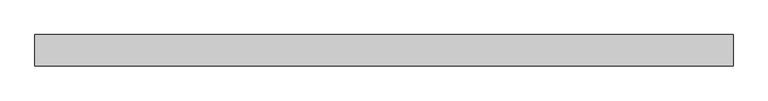
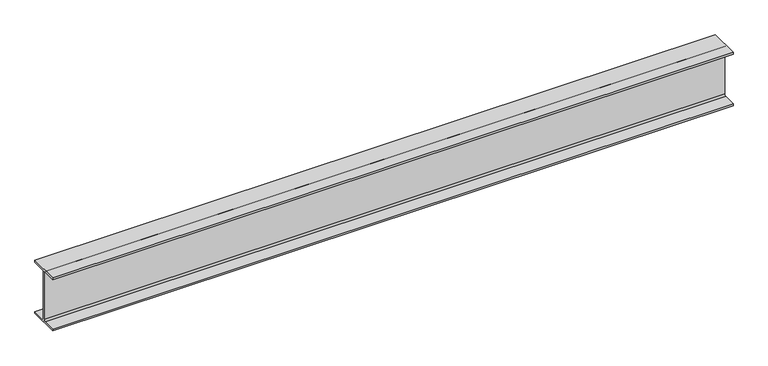
"""IFC4 building model written with IfcOpenShell, lengths in millimetres: beam geometry, Steel Beam_H-KSD3502 : H_SB_ASB_H-200x200x8x12."""

import ifcopenshell
import ifcopenshell.guid

model = None  # the IFC model being written
_history = None  # IfcOwnerHistory: only IFC2X3 demands one
_inside = {}  # id of a spatial element -> (the spatial element, [elements in it])
_under = {}  # id of a project, library or spatial element -> (it, [spatial elements below it])
_declared = {}  # id of a project -> (the project, [libraries it declares])
_typed = {}  # id of a type object -> (the type object, [elements of that type])
_made_of = {}  # id of a material, layer set ... -> (it, [elements and type objects made of it])


def new_model(schema):
    """Start an empty IFC model of exactly this schema.

    Asked for "IFC4X3", IfcOpenShell would pick the latest addendum, in which some entities
    have other attributes; the version numbers below select the first issue.
    IFC2X3 requires an IfcOwnerHistory on every rooted entity: one is made here for all.
    """
    global model, _history
    if schema == "IFC4X3":
        model = ifcopenshell.file(schema_version=(4, 3, 0, 0))
    else:
        model = ifcopenshell.file(schema=schema)
    _inside.clear()
    _under.clear()
    _declared.clear()
    _typed.clear()
    _made_of.clear()
    _history = None
    if model.schema == "IFC2X3":
        org = make("IfcOrganization", Name="unknown")
        user = make(
            "IfcPersonAndOrganization",
            ThePerson=make("IfcPerson", FamilyName="unknown"),
            TheOrganization=org,
        )
        app = make(
            "IfcApplication",
            ApplicationDeveloper=org,
            Version="unknown",
            ApplicationFullName="unknown",
            ApplicationIdentifier="unknown",
        )
        _history = make(
            "IfcOwnerHistory",
            OwningUser=user,
            OwningApplication=app,
            ChangeAction="ADDED",
            CreationDate=0,
        )
    return model


def make(cls, **values):
    """One entity of the class cls with the attributes given. An attribute that is None is left unset."""
    return model.create_entity(
        cls, **{name: value for name, value in values.items() if value is not None}
    )


def rooted(cls, **values):
    """An entity with a GlobalId (a new one), such as an element, a storey or a relation."""
    return make(cls, GlobalId=ifcopenshell.guid.new(), OwnerHistory=_history, **values)


def si_unit(unit_type, name, prefix=None):
    """IfcSIUnit, for example si_unit("LENGTHUNIT", "METRE", prefix="MILLI")."""
    return make("IfcSIUnit", UnitType=unit_type, Prefix=prefix, Name=name)


def assignment(units):
    """IfcUnitAssignment: the units of a project."""
    return None if units is None else make("IfcUnitAssignment", Units=units)


def point(xyz):
    """IfcCartesianPoint."""
    return None if xyz is None else make("IfcCartesianPoint", Coordinates=xyz)


def direction(xyz):
    """IfcDirection."""
    return None if xyz is None else make("IfcDirection", DirectionRatios=xyz)


def frame(location, z_axis=None, x_axis=None):
    """IfcAxis2Placement3D, a coordinate frame: its origin and axes. An axis left out is left unset."""
    return make(
        "IfcAxis2Placement3D",
        Location=point(location),
        Axis=direction(z_axis),
        RefDirection=direction(x_axis),
    )


def frame_2d(location, x_axis=None):
    """IfcAxis2Placement2D, a coordinate frame in the plane: its origin and x axis."""
    return make(
        "IfcAxis2Placement2D", Location=point(location), RefDirection=direction(x_axis)
    )


def origin():
    """The frame at (0, 0, 0) with its axes left unset."""
    return frame((0.0, 0.0, 0.0))


def place(relative_to, where):
    """IfcLocalPlacement: puts the frame where relative to a parent placement (None: the world)."""
    return make(
        "IfcLocalPlacement", PlacementRelTo=relative_to, RelativePlacement=where
    )


def context(
    kind, dimensions, precision=None, world=None, true_north=None, identifier=None
):
    """IfcGeometricRepresentationContext, for example the 3D "Model" context."""
    return make(
        "IfcGeometricRepresentationContext",
        ContextIdentifier=identifier,
        ContextType=kind,
        CoordinateSpaceDimension=dimensions,
        Precision=precision,
        WorldCoordinateSystem=world,
        TrueNorth=true_north,
    )


def project(units=None, contexts=None):
    """IfcProject with its units and contexts."""
    return rooted(
        "IfcProject",
        Name="project",
        RepresentationContexts=contexts,
        UnitsInContext=assignment(units),
    )


def spatial(cls, under=None, at=None, **own):
    """A site, building, storey or space (cls), placed at a placement, below another one or the project."""
    s = rooted(cls, ObjectPlacement=at, **own)
    if under is not None:
        _under.setdefault(under.id(), (under, []))[1].append(s)
    return s


def polyline(points):
    """IfcPolyline through the points."""
    return make("IfcPolyline", Points=[point(p) for p in points])


def circle_curve(where, radius):
    """IfcCircle in the frame where."""
    return make("IfcCircle", Position=where, Radius=radius)


def trimmed(basis, trim1, trim2, sense, master):
    """IfcTrimmedCurve: the piece of a basis curve between two trims."""
    return make(
        "IfcTrimmedCurve",
        BasisCurve=basis,
        Trim1=trim1,
        Trim2=trim2,
        SenseAgreement=sense,
        MasterRepresentation=master,
    )


def segment(curve, same_sense, transition):
    """IfcCompositeCurveSegment."""
    return make(
        "IfcCompositeCurveSegment",
        Transition=transition,
        SameSense=same_sense,
        ParentCurve=curve,
    )


def composite_curve(segments, self_intersect=None):
    """IfcCompositeCurve: segments joined end to end."""
    return make("IfcCompositeCurve", Segments=segments, SelfIntersect=self_intersect)


def outline(outer, holes=None, kind="AREA"):
    """IfcArbitraryClosedProfileDef: a profile drawn as a closed curve; with holes, ...WithVoids."""
    if holes is None:
        return make("IfcArbitraryClosedProfileDef", ProfileType=kind, OuterCurve=outer)
    return make(
        "IfcArbitraryProfileDefWithVoids",
        ProfileType=kind,
        OuterCurve=outer,
        InnerCurves=holes,
    )


def extrude(swept, where, along, depth):
    """IfcExtrudedAreaSolid: the profile swept, set in the frame where, extruded along a direction by depth."""
    return make(
        "IfcExtrudedAreaSolid",
        SweptArea=swept,
        Position=where,
        ExtrudedDirection=direction(along),
        Depth=depth,
    )


def shape(context_of_items, identifier, shape_type, items):
    """IfcShapeRepresentation: the items that make up one representation, for example the "Body"."""
    return make(
        "IfcShapeRepresentation",
        ContextOfItems=context_of_items,
        RepresentationIdentifier=identifier,
        RepresentationType=shape_type,
        Items=items,
    )


def source(mapping_origin, context_of_items, identifier, shape_type, items):
    """IfcRepresentationMap: a shape defined once, which mapped items show again and again."""
    return make(
        "IfcRepresentationMap",
        MappingOrigin=mapping_origin,
        MappedRepresentation=shape(context_of_items, identifier, shape_type, items),
    )


def transform(
    local_origin,
    x_axis=None,
    y_axis=None,
    z_axis=None,
    scale=None,
    scale2=None,
    scale3=None,
    uniform=True,
):
    """IfcCartesianTransformationOperator3D, or its non-uniform kind. x_axis, y_axis, z_axis: its Axis1, 2, 3."""
    if uniform:
        return make(
            "IfcCartesianTransformationOperator3D",
            Axis1=direction(x_axis),
            Axis2=direction(y_axis),
            LocalOrigin=point(local_origin),
            Scale=scale,
            Axis3=direction(z_axis),
        )
    return make(
        "IfcCartesianTransformationOperator3DnonUniform",
        Axis1=direction(x_axis),
        Axis2=direction(y_axis),
        LocalOrigin=point(local_origin),
        Scale=scale,
        Axis3=direction(z_axis),
        Scale2=scale2,
        Scale3=scale3,
    )


def mapped(mapping_source, mapping_target):
    """IfcMappedItem: shows the shape of a source again, moved by a transform."""
    return make(
        "IfcMappedItem", MappingSource=mapping_source, MappingTarget=mapping_target
    )


def made_of(thing, what):
    """Note that an element or type object is made of a material, layer set ...; save() writes the relation."""
    if what is not None:
        _made_of.setdefault(what.id(), (what, []))[1].append(thing)
    return thing


def element(
    cls,
    number,
    at=None,
    inside=None,
    cuts=None,
    type_object=None,
    material=None,
    context=None,
    identifier="Body",
    shape_type=None,
    held_by="IfcProductDefinitionShape",
    body=None,
    shapes=None,
    **own,
):
    """One element of the class cls, such as IfcWall. Its Tag is "e" and its number.

    at: its placement. inside: the storey or other place that contains it. cuts: it is an
    opening in that element (IfcRelVoidsElement). A single representation is given by context,
    identifier, shape_type and body (its items); several are given by shapes. held_by: the class
    of the entity that holds the representations. save() writes the other relations.
    """
    e = rooted(cls, Tag="e%d" % number, ObjectPlacement=at, **own)
    if body is not None:
        shapes = [shape(context, identifier, shape_type, body)]
    if shapes is not None:
        e.Representation = make(held_by, Representations=shapes)
    if inside is not None:
        _inside.setdefault(inside.id(), (inside, []))[1].append(e)
    if cuts is not None:
        rooted(
            "IfcRelVoidsElement", RelatingBuildingElement=cuts, RelatedOpeningElement=e
        )
    if type_object is not None:
        _typed.setdefault(type_object.id(), (type_object, []))[1].append(e)
    return made_of(e, material)


def aggregate(whole, parts):
    """IfcRelAggregates: a whole, such as a stair, and the parts it consists of."""
    return rooted("IfcRelAggregates", RelatingObject=whole, RelatedObjects=parts)


def save(model, path):
    """Write the relations noted so far, then the file.

    IfcRelAggregates (storeys below a building ...), IfcRelContainedInSpatialStructure (elements
    in a storey), IfcRelDefinesByType, IfcRelAssociatesMaterial and IfcRelDeclares: one each for
    every whole, place, type object, material and project.
    """
    for whole, parts in _under.values():
        aggregate(whole, parts)
    for where, things in _inside.values():
        rooted(
            "IfcRelContainedInSpatialStructure",
            RelatedElements=things,
            RelatingStructure=where,
        )
    for kind, things in _typed.values():
        rooted("IfcRelDefinesByType", RelatedObjects=things, RelatingType=kind)
    for what, things in _made_of.values():
        rooted("IfcRelAssociatesMaterial", RelatedObjects=things, RelatingMaterial=what)
    for by, libraries in _declared.values():
        rooted("IfcRelDeclares", RelatingContext=by, RelatedDefinitions=libraries)
    model.write(path)


def beam_fe90bdae(model_context):
    return source(origin(), model_context, "Body", "SweptSolid", [
        extrude(outline(composite_curve([segment(polyline([(82.5, -141.5), (82.5, -151.7), (-82.5, -151.7), (-82.5, -141.5), (-11.9, -141.5)]), True, "CONTINUOUS"), segment(trimmed(circle_curve(frame_2d((-11.9, -132.6)), 8.9), [point((-11.9, -141.5))], [point((-3.0, -132.6))], True, "CARTESIAN"), True, "CONTINUOUS"), segment(polyline([(-3.0, -132.6), (-3.0, 132.6)]), True, "CONTINUOUS"), segment(trimmed(circle_curve(frame_2d((-11.9, 132.6)), 8.9), [point((-3.0, 132.6))], [point((-11.9, 141.5))], True, "CARTESIAN"), True, "CONTINUOUS"), segment(polyline([(-11.9, 141.5), (-82.5, 141.5), (-82.5, 151.7), (82.5, 151.7), (82.5, 141.5), (11.9, 141.5)]), True, "CONTINUOUS"), segment(trimmed(circle_curve(frame_2d((11.9, 132.6)), 8.9), [point((11.9, 141.5))], [point((3.0, 132.6))], True, "CARTESIAN"), True, "CONTINUOUS"), segment(polyline([(3.0, 132.6), (3.0, -132.6)]), True, "CONTINUOUS"), segment(trimmed(circle_curve(frame_2d((11.9, -132.6)), 8.9), [point((3.0, -132.6))], [point((11.9, -141.5))], True, "CARTESIAN"), True, "CONTINUOUS"), segment(polyline([(11.9, -141.5), (82.5, -141.5)]), True, "CONTINUOUS")], self_intersect=False)), frame((-1848.779151, 0.0, 0.0), z_axis=(1.0, 0.0, 0.0), x_axis=(0.0, 1.0, 0.0)), (0.0, 0.0, 1.0), 3672.4688696),
    ])


if __name__ == "__main__":
    model = new_model("IFC4")
    model_context = context("Model", 3, world=origin())
    ifc_project = project(units=[si_unit("LENGTHUNIT", "METRE", prefix="MILLI")], contexts=[model_context])
    site = spatial("IfcSite", under=ifc_project)
    building = spatial("IfcBuilding", under=site)
    placement = place(None, origin())
    beam_shape = beam_fe90bdae(model_context)
    element("IfcBeam", 1, ObjectType="Steel Beam_H-KSD3502 : H_SB_ASB_H-200x200x8x12", at=placement, inside=building, context=model_context, shape_type="MappedRepresentation", body=[
        mapped(beam_shape, transform((0.0, 0.0, 0.0), x_axis=(1.0, 0.0, 0.0), y_axis=(0.0, 1.0, 0.0), z_axis=(0.0, 0.0, 1.0))),
    ])
    save(model, "model.ifc")

# Revit data of these elements
# Type "Steel Beam_H-KSD3502 : H_SB_ASB_H-200x200x8x12"
#   Width = 20.0 cm
#   Web Thickness = 0.8 cm
#   Web Fillet = 1.3 cm
#   Warping Constant = 141376.0 cm⁶
#   Torsional Moment of Inertia = 26.2485 cm⁴
#   Torsional Modulus = 1.0 cm³
#   Section Area = 63.53 cm²
#   Plastic Modulus weak axis = 244.0 cm³
#   Plastic Modulus strong axis = 525.0 cm³
#   Perimeter = 1.16 m²/m
#   Nominal Weight = 49.90 kgf/m
#   Moment of Inertia weak axis = 1600.00 cm⁴
#   Moment of Inertia strong axis = 4720.00 cm⁴
#   Height = 20.0 cm
#   Flange Thickness = 1.2 cm
#   Elastic Modulus weak axis = 160.0 cm³
#   Elastic Modulus strong axis = 472.0 cm³
#   Centroid Vertical = 10.0 cm
#   Centroid Horizontal = 10.0 cm
#   Length [instance default] = 1.5240 m
#   Structural Material [instance default] = Steel, 45-345
#   Assembly Code = ""
# Element 1 (IfcBeam, "Steel Beam_H-KSD3502 : H_SB_ASB_H-200x200x8x12")
#   Structural Material = none
# Materials
#   "Steel, 45-345": class "Metal", colour RGB 189 187 185, transparency 0, Description = "Steel 345 MPa", Cost = 0
